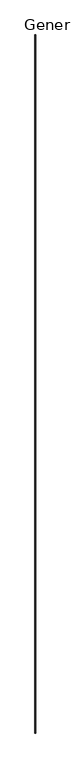
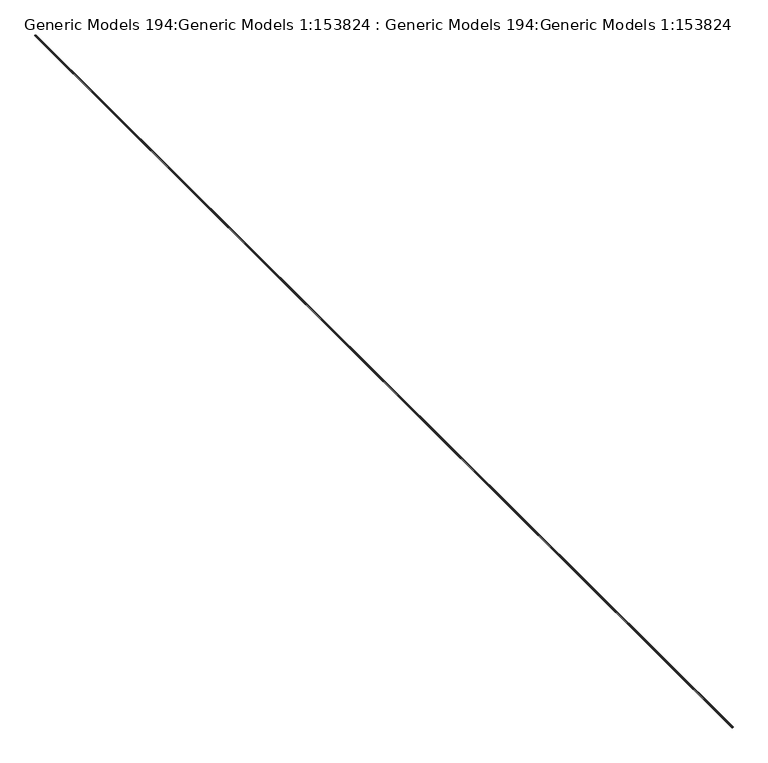
"""IFC4 building model written with IfcOpenShell, lengths in millimetres: proxy geometry, Generic Models 194:Generic Models 1:153824 : Generic Models 194:Generic Models 1:153824."""

from ifc_helpers import new_model, si_unit, point, frame, frame_2d, origin, place, context, project, spatial, polyline, circle_curve, trimmed, segment, composite_curve, outline, extrude, source, transform, mapped, element, save


def generic_models_194_generic_models_1_153824_generic_models_6c1c568c(model_context):
    return source(origin(), model_context, "Body", "SweptSolid", [
        extrude(outline(composite_curve([segment(trimmed(circle_curve(frame_2d((5926.0064027, -5366.526502)), 6.4650413), [point((5930.7689027, -5362.1543913))], [point((5921.2439027, -5362.1543913))], True, "CARTESIAN"), True, "CONTINUOUS"), segment(polyline([(5921.2439027, -5362.1543913), (5921.2439027, -5357.3918913)]), True, "CONTINUOUS"), segment(trimmed(circle_curve(frame_2d((5926.0064027, -5361.764002)), 6.4650413), [point((5921.2439027, -5357.3918913))], [point((5923.1498906, -5355.9642523))], False, "CARTESIAN"), True, "CONTINUOUS"), segment(polyline([(5923.1498906, -5355.9642523), (5922.3956562, -5354.9063395), (5921.8111677, -5353.6294386), (5921.4239028, -5352.1935785), (5921.2520672, -5350.6662608), (5921.3037391, -5349.1192868), (5921.5764895, -5347.6253818), (5922.0574958, -5346.2547761), (5922.7241455, -5345.0719037), (5923.5450984, -5344.1323731), (5924.4817604, -5343.4803527), (5925.4900979, -5343.146495), (5926.5227076, -5343.146495), (5927.531045, -5343.4803527), (5928.4677071, -5344.1323731), (5929.28866, -5345.0719037), (5929.9553097, -5346.2547761), (5930.436316, -5347.6253818), (5930.7090664, -5349.1192868), (5930.7607383, -5350.6662608), (5930.5889027, -5352.1935785), (5930.2016377, -5353.6294386), (5929.6171493, -5354.9063395), (5928.8629149, -5355.9642523)]), True, "CONTINUOUS"), segment(trimmed(circle_curve(frame_2d((5926.0064027, -5361.764002)), 6.4650413), [point((5928.8629149, -5355.9642523))], [point((5930.7689027, -5357.3918913))], False, "CARTESIAN"), True, "CONTINUOUS"), segment(polyline([(5930.7689027, -5357.3918913), (5930.7689027, -5362.1543913)]), True, "CONTINUOUS")], self_intersect=False)), frame((0.0, -6877.9974793, 0.0), z_axis=(0.0, 1.0, 0.0), x_axis=(0.0, 0.0, 1.0)), (0.0, 0.0, 1.0), 19050.0),
    ])


if __name__ == "__main__":
    model = new_model("IFC4")
    model_context = context("Model", 3, world=origin())
    ifc_project = project(units=[si_unit("LENGTHUNIT", "METRE", prefix="MILLI")], contexts=[model_context])
    site = spatial("IfcSite", under=ifc_project)
    building = spatial("IfcBuilding", under=site)
    placement = place(None, origin())
    generic_models_194_generic_models_1_153824_generic_models_shape = generic_models_194_generic_models_1_153824_generic_models_6c1c568c(model_context)
    element("IfcBuildingElementProxy", 1, Name="Generic Models 194:Generic Models 1:153824 : Generic Models 194:Generic Models 1:153824", ObjectType="Generic Models 194:Generic Models 1:153824 : Generic Models 194:Generic Models 1:153824", at=placement, inside=building, context=model_context, shape_type="MappedRepresentation", body=[
        mapped(generic_models_194_generic_models_1_153824_generic_models_shape, transform((0.0, 0.0, 0.0), x_axis=(1.0, 0.0, 0.0), y_axis=(0.0, 1.0, 0.0), z_axis=(0.0, 0.0, 1.0))),
    ])
    save(model, "model.ifc")

# Revit data of these elements
# Type "Generic Models 194:Generic Models 1:153824 : Generic Models 194:Generic Models 1:153824"
#   NameOverride = "Generic Models 194:Generic Models 1:153824"
#   ObjectTypeOverride = "Generic Models 194:Generic Models 1"
#   Reference = "Generic Models 1"
#   Category = "Generic Models"
#   Tag = "153824"
# Element 1 (IfcBuildingElementProxy, "Generic Models 194:Generic Models 1:153824 : Generic Models 194:Generic Models 1:153824")
#   Materials on its faces: "_SEALANT AND BACKROD, IF NECESSARY 12051"
# Materials
#   "_SEALANT AND BACKROD, IF NECESSARY 12051": class "Unassigned", colour RGB 190 220 196, transparency 0
